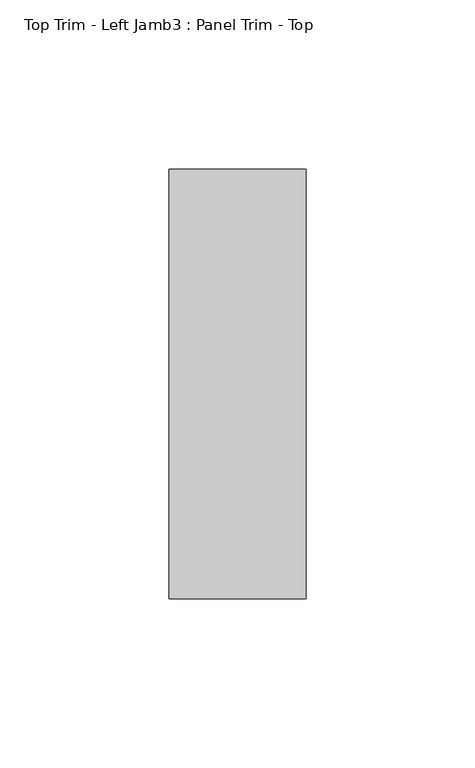
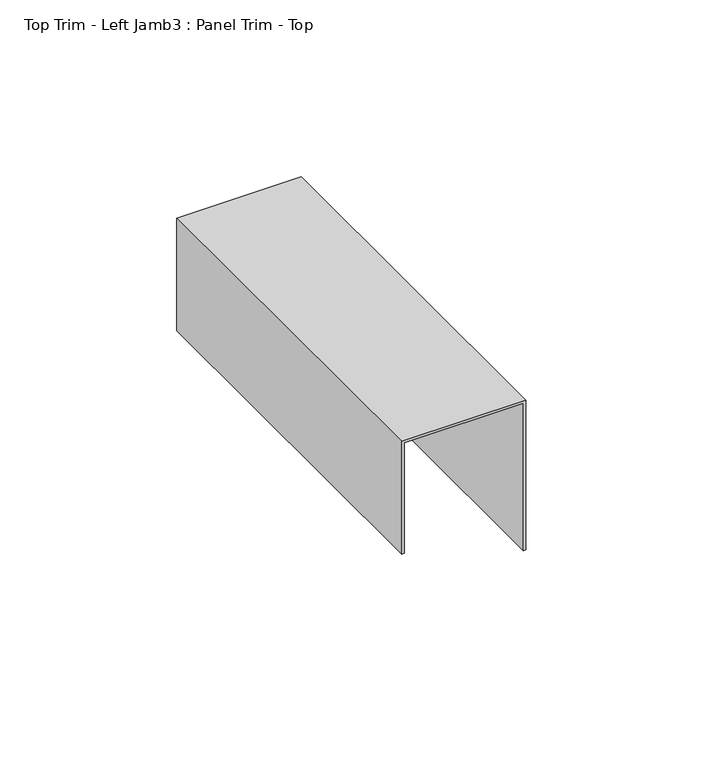
"""IFC4 building model written with IfcOpenShell, lengths in millimetres: proxy geometry, Top Trim - Left Jamb3 : Panel Trim - Top."""

from ifc_helpers import new_model, si_unit, frame, origin, place, context, project, spatial, polyline, outline, extrude, source, transform, mapped, element, save


def top_trim_left_jamb3_panel_trim_top_a1816676(model_context):
    return source(origin(), model_context, "Body", "SweptSolid", [
        extrude(outline(polyline([(2438.4, 587327.0060739), (2438.4, 587365.8934739), (2387.6, 587365.8934739), (2387.6, 587366.6808739), (2439.19375, 587366.6808739), (2439.19375, 587326.2186739), (2400.3, 587326.2186739), (2400.3, 587327.0060739), (2438.4, 587327.0060739)])), frame((0.0, -536420.7663841, 0.0), z_axis=(0.0, 1.0, 0.0), x_axis=(0.0, 0.0, 1.0)), (0.0, 0.0, 1.0), 127.0),
    ])


if __name__ == "__main__":
    model = new_model("IFC4")
    model_context = context("Model", 3, world=origin())
    ifc_project = project(units=[si_unit("LENGTHUNIT", "METRE", prefix="MILLI")], contexts=[model_context])
    site = spatial("IfcSite", under=ifc_project)
    building = spatial("IfcBuilding", under=site)
    placement = place(None, origin())
    top_trim_left_jamb3_panel_trim_top_shape = top_trim_left_jamb3_panel_trim_top_a1816676(model_context)
    element("IfcBuildingElementProxy", 1, Name="Top Trim - Left Jamb3 : Panel Trim - Top", ObjectType="Top Trim - Left Jamb3 : Panel Trim - Top", at=placement, inside=building, context=model_context, shape_type="MappedRepresentation", body=[
        mapped(top_trim_left_jamb3_panel_trim_top_shape, transform((0.0, 0.0, 0.0), x_axis=(1.0, 0.0, 0.0), y_axis=(0.0, 1.0, 0.0), z_axis=(0.0, 0.0, 1.0))),
    ])
    save(model, "model.ifc")

# Revit data of these elements
# Element 1 (IfcBuildingElementProxy, "Top Trim - Left Jamb3 : Panel Trim - Top")
#   Materials on its faces: "EDGE TRIM BY MTL PANEL MFR."
# Materials
#   "EDGE TRIM BY MTL PANEL MFR.": class "Generic", colour RGB 239 242 240, transparency 0, Cost = 0
